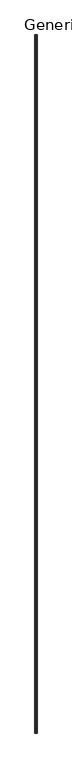
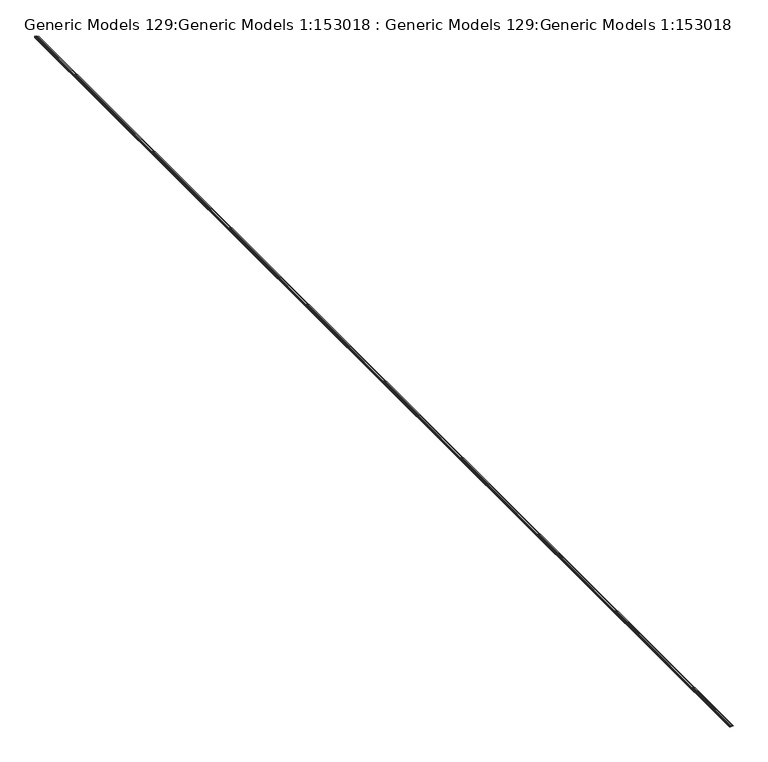
"""IFC4 building model written with IfcOpenShell, lengths in millimetres: proxy geometry, Generic Models 129:Generic Models 1:153018 : Generic Models 129:Generic Models 1:153018."""

from ifc_helpers import new_model, si_unit, frame, origin, place, context, project, spatial, polyline, outline, extrude, source, transform, mapped, element, save


def generic_models_129_generic_models_1_153018_generic_models_b2cb1f58(model_context):
    return source(origin(), model_context, "Body", "SweptSolid", [
        extrude(outline(polyline([(3046.095, 7053.458213), (3046.095, 7033.773213), (3048.3048, 7033.773213), (3048.3048, 7034.6320539), (3068.6193787, 7034.6320539), (3068.6193787, 7033.3620539), (3049.5748, 7033.3620539), (3049.5748, 7032.503213), (3044.825, 7032.503213), (3044.825, 7054.728213), (3056.255, 7054.728213), (3056.255, 7067.428213), (3044.825, 7067.428213), (3044.825, 7091.141397), (3046.095, 7091.141397), (3046.095, 7068.698213), (3057.525, 7068.698213), (3057.525, 7053.458213), (3046.095, 7053.458213)])), frame((0.0, -6877.9974793, 0.0), z_axis=(0.0, 1.0, 0.0), x_axis=(0.0, 0.0, 1.0)), (0.0, 0.0, 1.0), 19050.0),
    ])


if __name__ == "__main__":
    model = new_model("IFC4")
    model_context = context("Model", 3, world=origin())
    ifc_project = project(units=[si_unit("LENGTHUNIT", "METRE", prefix="MILLI")], contexts=[model_context])
    site = spatial("IfcSite", under=ifc_project)
    building = spatial("IfcBuilding", under=site)
    placement = place(None, origin())
    generic_models_129_generic_models_1_153018_generic_models_shape = generic_models_129_generic_models_1_153018_generic_models_b2cb1f58(model_context)
    element("IfcBuildingElementProxy", 1, Name="Generic Models 129:Generic Models 1:153018 : Generic Models 129:Generic Models 1:153018", ObjectType="Generic Models 129:Generic Models 1:153018 : Generic Models 129:Generic Models 1:153018", at=placement, inside=building, context=model_context, shape_type="MappedRepresentation", body=[
        mapped(generic_models_129_generic_models_1_153018_generic_models_shape, transform((0.0, 0.0, 0.0), x_axis=(1.0, 0.0, 0.0), y_axis=(0.0, 1.0, 0.0), z_axis=(0.0, 0.0, 1.0))),
    ])
    save(model, "model.ifc")

# Revit data of these elements
# Type "Generic Models 129:Generic Models 1:153018 : Generic Models 129:Generic Models 1:153018"
#   NameOverride = "Generic Models 129:Generic Models 1:153018"
#   ObjectTypeOverride = "Generic Models 129:Generic Models 1"
#   Reference = "Generic Models 1"
#   Category = "Generic Models"
#   Tag = "153018"
# Element 1 (IfcBuildingElementProxy, "Generic Models 129:Generic Models 1:153018 : Generic Models 129:Generic Models 1:153018")
#   Materials on its faces: "_16 GA. COPPER SOFFIT DRIP SCREED 1359"
# Materials
#   "_16 GA. COPPER SOFFIT DRIP SCREED 1359": class "Unassigned", colour RGB 253 192 103, transparency 0
